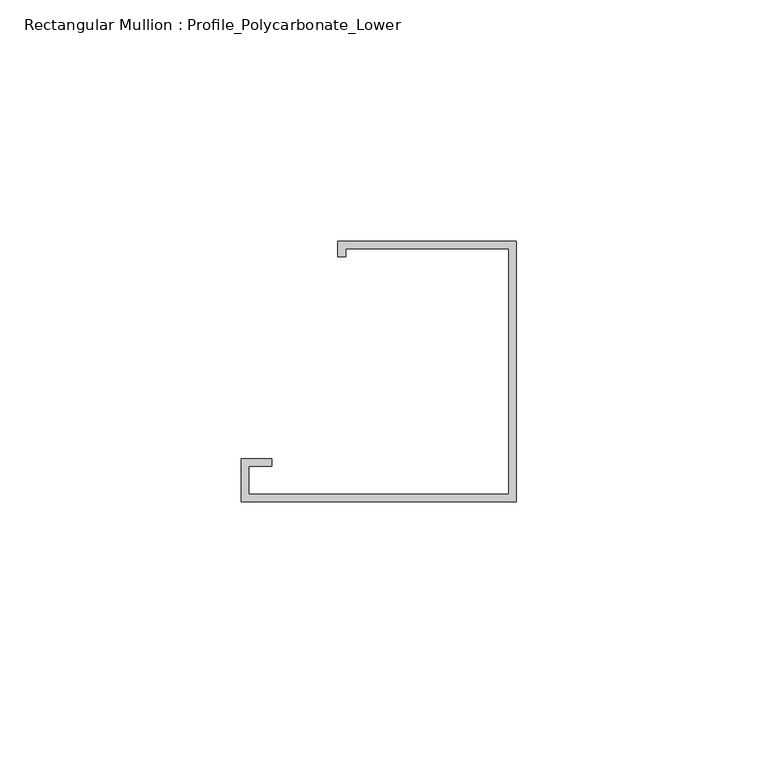
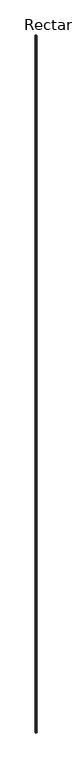
"""IFC4 building model written with IfcOpenShell, lengths in millimetres: member geometry, Rectangular Mullion : Profile_Polycarbonate_Lower."""

from ifc_helpers import new_model, si_unit, frame, origin, place, context, project, spatial, polyline, outline, extrude, source, transform, mapped, element, save


def rectangular_mullion_profile_polycarbonate_lower_fe460ce4(model_context):
    return source(origin(), model_context, "Body", "SweptSolid", [
        extrude(outline(polyline([(0.0, -28.984575), (-56.9976, -28.984575), (-56.9976, -19.992975), (-50.6476, -19.992975), (-50.6476, -21.580475), (-55.4101, -21.580475), (-55.4101, -27.397075), (-1.5875, -27.397075), (-1.5875, 23.428325), (-35.3949, 23.428325), (-35.3949, 21.840825), (-36.9824, 21.840825), (-36.9824, 25.015825), (0.0, 25.015825), (0.0, -28.984575)])), frame((0.0, 0.0, -29419.55), z_axis=(0.0, 0.0, 1.0), x_axis=(1.0, 0.0, 0.0)), (0.0, 0.0, 1.0), 29419.55),
    ])


if __name__ == "__main__":
    model = new_model("IFC4")
    model_context = context("Model", 3, world=origin())
    ifc_project = project(units=[si_unit("LENGTHUNIT", "METRE", prefix="MILLI")], contexts=[model_context])
    site = spatial("IfcSite", under=ifc_project)
    building = spatial("IfcBuilding", under=site)
    placement = place(None, origin())
    rectangular_mullion_profile_polycarbonate_lower_shape = rectangular_mullion_profile_polycarbonate_lower_fe460ce4(model_context)
    element("IfcMember", 1, ObjectType="Rectangular Mullion : Profile_Polycarbonate_Lower", at=placement, inside=building, context=model_context, shape_type="MappedRepresentation", body=[
        mapped(rectangular_mullion_profile_polycarbonate_lower_shape, transform((0.0, 0.0, 0.0), x_axis=(1.0, 0.0, 0.0), y_axis=(0.0, 1.0, 0.0), z_axis=(0.0, 0.0, 1.0))),
    ])
    save(model, "model.ifc")

# Revit data of these elements
# Type "Rectangular Mullion : Profile_Polycarbonate_Lower"
#   built-in parameter 1007322 = 0.177167 (stored number, unit not read)
#   built-in parameter 1007321 = 0 (stored number, unit not read)
#   built-in parameter 1007320 = 0.00520833 (stored number, unit not read)
